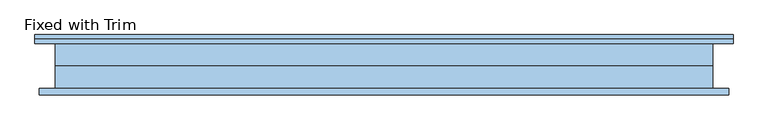
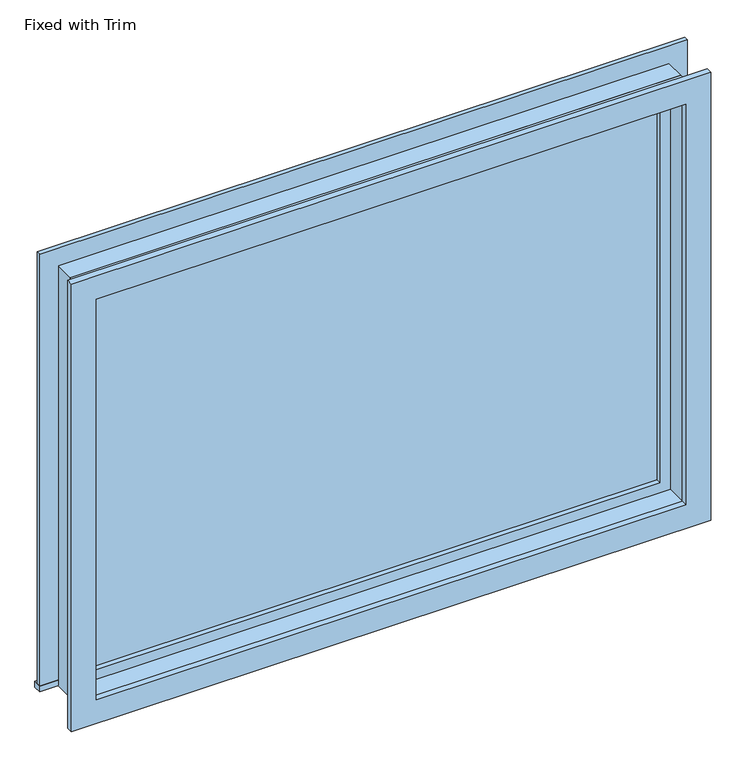
"""IFC4 building model written with IfcOpenShell, lengths in millimetres: window geometry, Fixed with Trim."""

from ifc_helpers import new_model, si_unit, frame, origin, place, context, project, spatial, polyline, outline, extrude, source, transform, mapped, element, save


def fixed_with_trim_b7b04b7d(model_context):
    return source(origin(), model_context, "Body", "SweptSolid", [
        extrude(outline(polyline([(-1028.7, 88.9), (952.5, 88.9), (952.5, 63.5), (-1028.7, 63.5), (-1028.7, 88.9)])), frame((0.0, 0.0, 914.4), z_axis=(0.0, 0.0, 1.0), x_axis=(1.0, 0.0, 0.0)), (0.0, 0.0, 1.0), 19.05),
        extrude(outline(polyline([(2254.25, -952.5), (2254.25, 876.3), (933.45, 876.3), (933.45, 952.5), (2330.45, 952.5), (2330.45, -1028.7), (933.45, -1028.7), (933.45, -952.5), (2254.25, -952.5)])), frame((0.0, 63.5, 0.0), z_axis=(0.0, 1.0, 0.0), x_axis=(0.0, 0.0, 1.0)), (0.0, 0.0, 1.0), 12.7),
        extrude(outline(polyline([(2317.75, 939.8), (2317.75, -1016.0), (869.95, -1016.0), (869.95, 939.8), (2317.75, 939.8)]), holes=[polyline([(2241.55, 863.6), (946.15, 863.6), (946.15, -939.8), (2241.55, -939.8), (2241.55, 863.6)])]), frame((0.0, -82.55, 0.0), z_axis=(0.0, 1.0, 0.0), x_axis=(0.0, 0.0, 1.0)), (0.0, 0.0, 1.0), 19.05),
        extrude(outline(polyline([(831.85, 15.875), (-908.05, 15.875), (-908.05, 28.575), (831.85, 28.575), (831.85, 15.875)])), frame((0.0, 0.0, 977.9), z_axis=(0.0, 0.0, 1.0), x_axis=(1.0, 0.0, 0.0)), (0.0, 0.0, 1.0), 1231.9),
        extrude(outline(polyline([(2254.25, -952.5), (933.45, -952.5), (933.45, 876.3), (2254.25, 876.3), (2254.25, -952.5)]), holes=[polyline([(2209.8, -908.05), (2209.8, 831.85), (977.9, 831.85), (977.9, -908.05), (2209.8, -908.05)])]), frame((0.0, 0.0, 0.0), z_axis=(0.0, 1.0, 0.0), x_axis=(0.0, 0.0, 1.0)), (0.0, 0.0, 1.0), 44.45),
        extrude(outline(polyline([(2273.3, -971.55), (914.4, -971.55), (914.4, 895.35), (2273.3, 895.35), (2273.3, -971.55)]), holes=[polyline([(2241.55, -939.8), (2241.55, 863.6), (946.15, 863.6), (946.15, -939.8), (2241.55, -939.8)])]), frame((0.0, -63.5, 0.0), z_axis=(0.0, 1.0, 0.0), x_axis=(0.0, 0.0, 1.0)), (0.0, 0.0, 1.0), 63.5),
        extrude(outline(polyline([(2273.3, 895.35), (2273.3, -971.55), (914.4, -971.55), (914.4, 895.35), (2273.3, 895.35)]), holes=[polyline([(2254.25, 876.3), (933.45, 876.3), (933.45, -952.5), (2254.25, -952.5), (2254.25, 876.3)])]), frame((0.0, 0.0, 0.0), z_axis=(0.0, 1.0, 0.0), x_axis=(0.0, 0.0, 1.0)), (0.0, 0.0, 1.0), 63.5),
    ])


if __name__ == "__main__":
    model = new_model("IFC4")
    model_context = context("Model", 3, world=origin())
    ifc_project = project(units=[si_unit("LENGTHUNIT", "METRE", prefix="MILLI")], contexts=[model_context])
    site = spatial("IfcSite", under=ifc_project)
    building = spatial("IfcBuilding", under=site)
    placement = place(None, origin())
    fixed_with_trim_shape = fixed_with_trim_b7b04b7d(model_context)
    element("IfcWindow", 1, ObjectType="Fixed with Trim : 6'  1 1/2\" x 4'-5 1/2\"", at=placement, inside=building, context=model_context, shape_type="MappedRepresentation", body=[
        mapped(fixed_with_trim_shape, transform((0.0, 0.0, 0.0), x_axis=(1.0, 0.0, 0.0), y_axis=(0.0, 1.0, 0.0), z_axis=(0.0, 0.0, 1.0))),
    ])
    save(model, "model.ifc")

# Revit data of these elements
# Type "Fixed with Trim : 6'  1 1/2\" x 4'-5 1/2\""
#   Type Mark = "68"
#   Construction Type Id = "GSP4R"
#   Assembly Code = "B2020100"
#   Analytic Construction = "1/8 in Pilkington single glazing"
#   Visual Light Transmittance = 0.9
#   Solar Heat Gain Coefficient = 0.78
#   Heat Transfer Coefficient (U) = 3.6886 W/(m²·K)
#   Height = 4' - 5 1/2"
#   Default Sill Height = 3' - 0"
#   Trim Projection - Ext. = 0' - 0 1/2"
#   Trim Projection - Int. = 0' - 0 3/4"
#   Trim Width - Exterior = 0' - 3"
#   Trim Width - Interior = 0' - 3"
#   Width = 6' - 1 1/2"
#   Window Inset = 0' - 0 3/4"
#   Glass Pane Material = EXISTING WINDOW
#   Sash Material = Trim
#   Trim Exterior Material = Trim
#   Trim Interior Material = Trim
#   Wall Closure = (empty or 0)
# Element 1 (IfcWindow, "Fixed with Trim : 6'  1 1/2\" x 4'-5 1/2\"")
#   Materials on its faces: "Trim", "EXISTING WINDOW"
# Materials
#   "EXISTING WINDOW": class "Glass", colour RGB 218 227 224, transparency 0.85, Description = "Soda Lime Glass", Cost = 0
#   "Trim": class "Wood", colour RGB 250 251 245, transparency 0, Cost = 0
